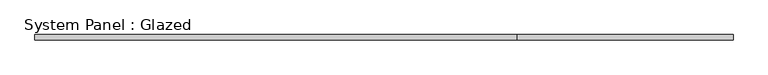
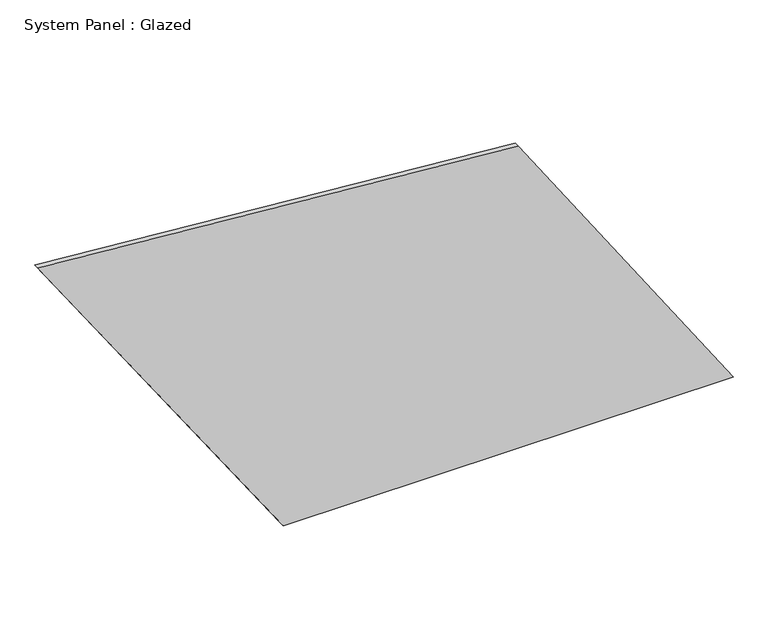
"""IFC4 building model written with IfcOpenShell, lengths in millimetres: plate geometry, System Panel : Glazed."""

from ifc_helpers import new_model, si_unit, frame, origin, place, context, project, spatial, polyline, outline, extrude, source, transform, mapped, element, save


def system_panel_glazed_399b75b5(model_context):
    return source(origin(), model_context, "Body", "SweptSolid", [
        extrude(outline(polyline([(0.0, -479.6873226), (0.0, 1628.9680699), (1497.2423052, 621.6714603), (1681.2371621, -1628.9680699), (0.0, -479.6873226)])), frame((0.0, -49.5, 0.0), z_axis=(0.0, 1.0, 0.0), x_axis=(0.0, 0.0, 1.0)), (0.0, 0.0, 1.0), 25.0),
    ])


if __name__ == "__main__":
    model = new_model("IFC4")
    model_context = context("Model", 3, world=origin())
    ifc_project = project(units=[si_unit("LENGTHUNIT", "METRE", prefix="MILLI")], contexts=[model_context])
    site = spatial("IfcSite", under=ifc_project)
    building = spatial("IfcBuilding", under=site)
    placement = place(None, origin())
    system_panel_glazed_shape = system_panel_glazed_399b75b5(model_context)
    element("IfcPlate", 1, ObjectType="System Panel : Glazed", at=placement, inside=building, context=model_context, shape_type="MappedRepresentation", body=[
        mapped(system_panel_glazed_shape, transform((0.0, 0.0, 0.0), x_axis=(1.0, 0.0, 0.0), y_axis=(0.0, 1.0, 0.0), z_axis=(0.0, 0.0, 1.0))),
    ])
    save(model, "model.ifc")

# Revit data of these elements
# Element 1 (IfcPlate, "System Panel : Glazed")
#   Materials on its faces: "Glass, Clear Glazing"
# Materials
#   "Glass, Clear Glazing": class "Glass", colour RGB 247 249 248, transparency 0.85, Description = "Clear glazing", Cost = 0
